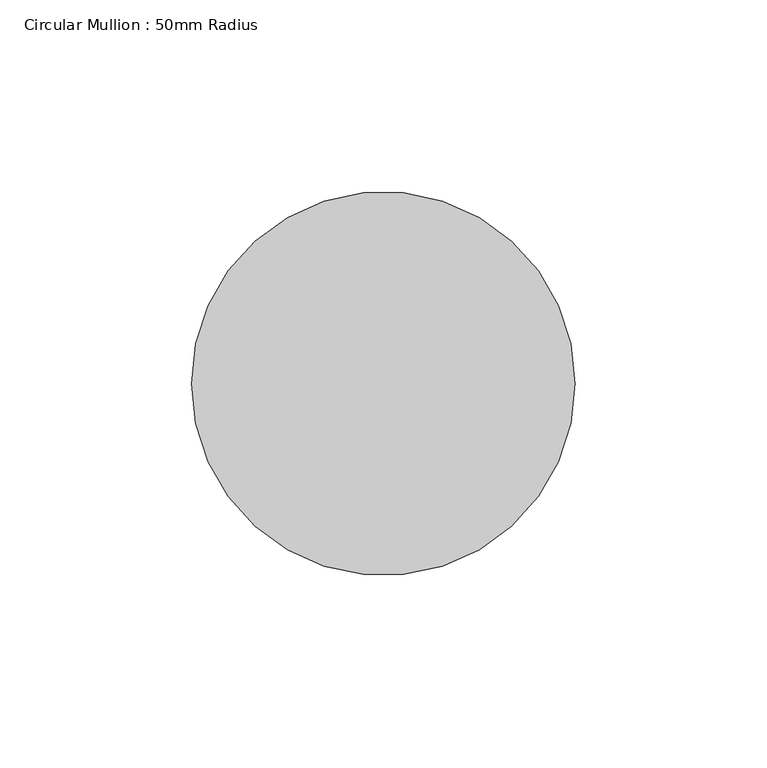
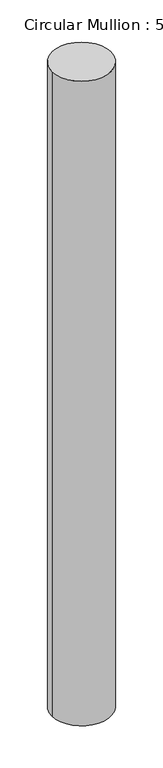
"""IFC4 building model written with IfcOpenShell, lengths in millimetres: member geometry, Circular Mullion : 50mm Radius."""

from ifc_helpers import new_model, si_unit, point, frame, origin, origin_2d, place, context, project, spatial, circle_curve, trimmed, segment, composite_curve, outline, extrude, source, transform, mapped, element, save


def circular_mullion_50mm_radius_b77ff1bc(model_context):
    return source(origin(), model_context, "Body", "SweptSolid", [
        extrude(outline(composite_curve([segment(trimmed(circle_curve(origin_2d(), 50.0), [point((50.0, 0.0))], [point((-50.0, 0.0))], False, "CARTESIAN"), True, "CONTINUOUS"), segment(trimmed(circle_curve(origin_2d(), 50.0), [point((-50.0, 0.0))], [point((50.0, 0.0))], False, "CARTESIAN"), True, "CONTINUOUS")], self_intersect=False)), frame((0.0, 0.0, -1148.0418669), z_axis=(0.0, 0.0, 1.0), x_axis=(1.0, 0.0, 0.0)), (0.0, 0.0, 1.0), 1148.0418669),
    ])


if __name__ == "__main__":
    model = new_model("IFC4")
    model_context = context("Model", 3, world=origin())
    ifc_project = project(units=[si_unit("LENGTHUNIT", "METRE", prefix="MILLI")], contexts=[model_context])
    site = spatial("IfcSite", under=ifc_project)
    building = spatial("IfcBuilding", under=site)
    placement = place(None, origin())
    circular_mullion_50mm_radius_shape = circular_mullion_50mm_radius_b77ff1bc(model_context)
    element("IfcMember", 1, ObjectType="Circular Mullion : 50mm Radius", at=placement, inside=building, context=model_context, shape_type="MappedRepresentation", body=[
        mapped(circular_mullion_50mm_radius_shape, transform((0.0, 0.0, 0.0), x_axis=(1.0, 0.0, 0.0), y_axis=(0.0, 1.0, 0.0), z_axis=(0.0, 0.0, 1.0))),
    ])
    save(model, "model.ifc")

# Revit data of these elements
# Type "Circular Mullion : 50mm Radius"
#   built-in parameter 1007350 = 0.164042 (stored number, unit not read)
# Element 1 (IfcMember, "Circular Mullion : 50mm Radius")
#   Materials on its faces: "Aluminium"
# Materials
#   "Aluminium": class "Metal", colour RGB 247 247 247, transparency 0, Description = "Aluminium 6061", Cost = 0
